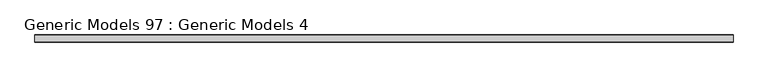
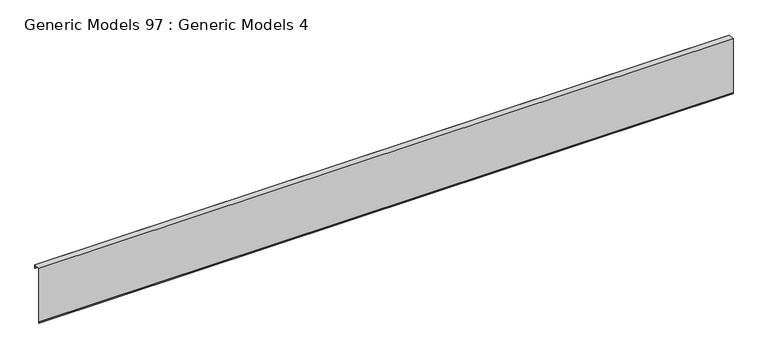
"""IFC4 building model written with IfcOpenShell, lengths in millimetres: proxy geometry, Generic Models 97 : Generic Models 4."""

from ifc_helpers import new_model, si_unit, frame, origin, place, context, project, spatial, polyline, outline, extrude, source, transform, mapped, element, save


def generic_models_97_generic_models_4_fb43a68a(model_context):
    return source(origin(), model_context, "Body", "SweptSolid", [
        extrude(outline(polyline([(7059.6509053, 127051.4250789), (7057.0550912, 127058.5570194), (7057.0550912, 127116.2640881), (6875.1408206, 127123.8438493), (6875.1408206, 125598.3569671), (6871.8967772, 125589.4440311), (6871.8967772, 125570.5614781), (6871.1030272, 125570.5614781), (6871.1030272, 125589.5839906), (6874.3470706, 125598.4969267), (6874.3470706, 127124.671361), (7057.8488412, 127117.0254539), (7057.8488412, 127058.696979), (7060.4446553, 127051.5650384), (7060.4446553, 127012.1744351), (7059.6509053, 127012.1744351), (7059.6509053, 127051.4250789)])), frame((-10234.5171316, 0.0, 0.0), z_axis=(1.0, 0.0, 0.0), x_axis=(0.0, 1.0, 0.0)), (0.0, 0.0, 1.0), 18643.6),
    ])


if __name__ == "__main__":
    model = new_model("IFC4")
    model_context = context("Model", 3, world=origin())
    ifc_project = project(units=[si_unit("LENGTHUNIT", "METRE", prefix="MILLI")], contexts=[model_context])
    site = spatial("IfcSite", under=ifc_project)
    building = spatial("IfcBuilding", under=site)
    placement = place(None, origin())
    generic_models_97_generic_models_4_shape = generic_models_97_generic_models_4_fb43a68a(model_context)
    element("IfcBuildingElementProxy", 1, Name="Generic Models 97 : Generic Models 4", ObjectType="Generic Models 97 : Generic Models 4", at=placement, inside=building, context=model_context, shape_type="MappedRepresentation", body=[
        mapped(generic_models_97_generic_models_4_shape, transform((0.0, 0.0, 0.0), x_axis=(1.0, 0.0, 0.0), y_axis=(0.0, 1.0, 0.0), z_axis=(0.0, 0.0, 1.0))),
    ])
    save(model, "model.ifc")

# Revit data of these elements
# Element 1 (IfcBuildingElementProxy, "Generic Models 97 : Generic Models 4")
#   Materials on its faces: "_(2) LAYERS NO. 30 ASTM D226 ASPHALT SATURATED ORGANIC FELT"
# Materials
#   "_(2) LAYERS NO. 30 ASTM D226 ASPHALT SATURATED ORGANIC FELT": class "Generic", colour RGB 67 154 161, transparency 0, Cost = 0
